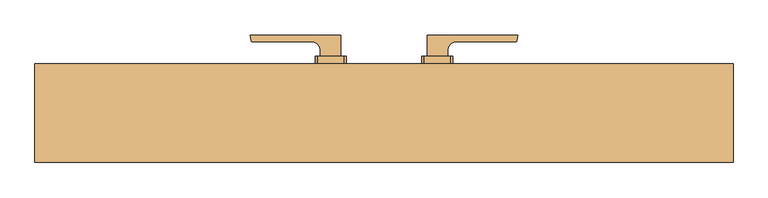
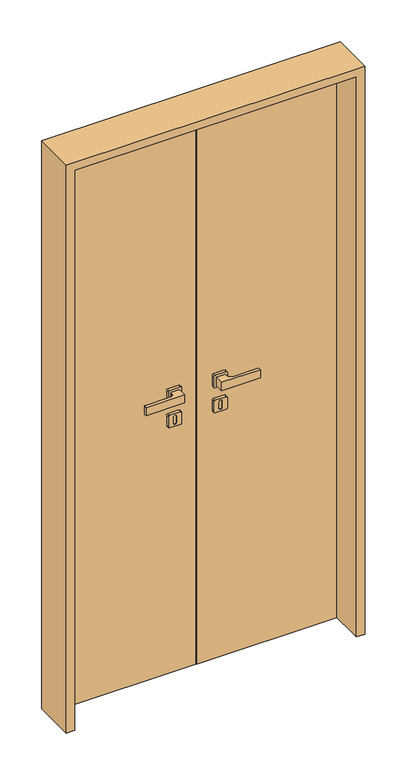
"""IFC4 building model written with IfcOpenShell, lengths in millimetres: door geometry, porta multiplas_growarq : porta giro duplo 50 cm_growarq."""

from ifc_helpers import new_model, si_unit, point, frame, frame_2d, origin, origin_with_axes, place, context, project, spatial, polyline, circle_curve, trimmed, segment, composite_curve, outline, extrude, source, transform, mapped, element, save
from ifc_brep_helpers import plane_surface, cylinder_surface, revolved_surface, advanced_brep


def door_77e2ac2a(model_context):
    return source(origin(), model_context, "Body", "SolidModel", [
        advanced_brep(
        [(-61.4752094, 86.0, 975.2140175), (-57.4752094, 86.0, 971.2140175), (-57.4752094, 86.0, 932.3348635), (-61.4752094, 86.0, 928.3348635), (-100.524804, 86.0, 928.3348635), (-104.524804, 86.0, 932.3348635), (-104.524804, 86.0, 971.2071442), (-100.5179308, 86.0, 975.2140175), (-75.9963765, 86.0, 963.1453546), (-86.0064486, 86.0, 963.1453546), (-86.0064486, 86.0, 940.4035264), (-75.9963765, 86.0, 940.4035264), (-61.4752094, 75.0, 975.2140175), (-100.5179308, 75.0, 975.2140175), (-104.524804, 75.0, 971.2071442), (-104.524804, 75.0, 932.3348635), (-100.524804, 75.0, 928.3348635), (-61.4752094, 75.0, 928.3348635), (-57.4752094, 75.0, 932.3348635), (-57.4752094, 75.0, 971.2140175), (-75.9963765, 84.0, 940.4035264), (-86.0064486, 84.0, 940.4035264), (-86.0064486, 84.0, 963.1453546), (-75.9963765, 84.0, 963.1453546)],
        [
            (0, 1, circle_curve(frame((-61.4752094, 86.0, 971.2140175), z_axis=(0.0, 1.0, 0.0), x_axis=(1.0, 0.0, 0.0)), 4.0)),
            (1, 2),
            (2, 3, circle_curve(frame((-61.4752094, 86.0, 932.3348635), z_axis=(0.0, 1.0, 0.0), x_axis=(1.0, 0.0, 0.0)), 4.0)),
            (3, 4),
            (4, 5, circle_curve(frame((-100.524804, 86.0, 932.3348635), z_axis=(0.0, 1.0, 0.0), x_axis=(1.0, 0.0, 0.0)), 4.0)),
            (5, 6),
            (6, 7, circle_curve(frame((-100.5179308, 86.0, 971.2071442), z_axis=(0.0, 1.0, 0.0), x_axis=(1.0, 0.0, 0.0)), 4.0068732)),
            (7, 0),
            (8, 9, circle_curve(frame((-81.0014126, 86.0, 963.1453546), z_axis=(0.0, -1.0, 0.0), x_axis=(1.0, 0.0, 0.0)), 5.0050361)),
            (9, 10),
            (10, 11, circle_curve(frame((-81.0014126, 86.0, 940.4035264), z_axis=(0.0, -1.0, 0.0), x_axis=(1.0, 0.0, 0.0)), 5.0050361)),
            (11, 8),
            (12, 13),
            (13, 14, circle_curve(frame((-100.5179308, 75.0, 971.2071442), z_axis=(0.0, -1.0, 0.0), x_axis=(1.0, 0.0, 0.0)), 4.0068732)),
            (14, 15),
            (15, 16, circle_curve(frame((-100.524804, 75.0, 932.3348635), z_axis=(0.0, -1.0, 0.0), x_axis=(1.0, 0.0, 0.0)), 4.0)),
            (16, 17),
            (17, 18, circle_curve(frame((-61.4752094, 75.0, 932.3348635), z_axis=(0.0, -1.0, 0.0), x_axis=(1.0, 0.0, 0.0)), 4.0)),
            (18, 19),
            (19, 12, circle_curve(frame((-61.4752094, 75.0, 971.2140175), z_axis=(0.0, -1.0, 0.0), x_axis=(1.0, 0.0, 0.0)), 4.0)),
            (7, 13),
            (12, 0),
            (6, 14),
            (5, 15),
            (4, 16),
            (3, 17),
            (2, 18),
            (1, 19),
            (20, 21, circle_curve(frame((-81.0014126, 84.0, 940.4035264), z_axis=(0.0, 1.0, 0.0), x_axis=(1.0, 0.0, 0.0)), 5.0050361)),
            (21, 22),
            (22, 23, circle_curve(frame((-81.0014126, 84.0, 963.1453546), z_axis=(0.0, 1.0, 0.0), x_axis=(1.0, 0.0, 0.0)), 5.0050361)),
            (23, 20),
            (23, 8),
            (11, 20),
            (21, 10),
            (9, 22),
        ],
        [
            plane_surface(frame((-100.5218961, 86.0, 975.2140175), z_axis=(0.0, 1.0, 0.0), x_axis=(-1.0, 0.0, 0.0))),
            plane_surface(frame((-100.5218961, 75.0, 975.2140175), z_axis=(0.0, -1.0, 0.0), x_axis=(1.0, 0.0, 0.0))),
            plane_surface(frame((-61.4752094, 86.0, 975.2140175), z_axis=(0.0, 0.0, 1.0), x_axis=(0.0, -1.0, 0.0))),
            cylinder_surface(frame((-100.5179308, 75.0, 971.2071442), z_axis=(0.0, 1.0, 0.0), x_axis=(1.0, 0.0, 0.0)), 4.0068732),
            plane_surface(frame((-104.524804, 86.0, 971.2071442), z_axis=(-1.0, 0.0, 0.0), x_axis=(0.0, -1.0, 0.0))),
            cylinder_surface(frame((-100.524804, 75.0, 932.3348635), z_axis=(0.0, 1.0, 0.0), x_axis=(1.0, 0.0, 0.0)), 4.0),
            plane_surface(frame((-100.524804, 86.0, 928.3348635), z_axis=(0.0, 0.0, -1.0), x_axis=(0.0, -1.0, 0.0))),
            cylinder_surface(frame((-61.4752094, 75.0, 932.3348635), z_axis=(0.0, 1.0, 0.0), x_axis=(1.0, 0.0, 0.0)), 4.0),
            plane_surface(frame((-57.4752094, 86.0, 932.3348635), z_axis=(1.0, 0.0, 0.0), x_axis=(0.0, -1.0, 0.0))),
            cylinder_surface(frame((-61.4752094, 75.0, 971.2140175), z_axis=(0.0, 1.0, 0.0), x_axis=(1.0, 0.0, 0.0)), 4.0),
            plane_surface(frame((-75.9963765, 84.0, 952.9958878), z_axis=(0.0, 1.0, 0.0), x_axis=(0.0, 0.0, -1.0))),
            plane_surface(frame((-75.9963765, 86.0, 940.4035264), z_axis=(-1.0, 0.0, 0.0), x_axis=(0.0, -1.0, 0.0))),
            plane_surface(frame((-86.0064486, 86.0, 963.1453546), z_axis=(1.0, 0.0, 0.0), x_axis=(0.0, -1.0, 0.0))),
            revolved_surface(polyline([(-75.9963765, 86.0, 940.4035264), (-75.9963765, 84.0, 940.4035264)]), (-81.0014126, 84.0, 940.4035264), (0.0, 1.0, 0.0)),
            revolved_surface(polyline([(-75.9963765, 86.0, 963.1453546), (-75.9963765, 84.0, 963.1453546)]), (-81.0014126, 84.0, 963.1453546), (0.0, 1.0, 0.0)),
        ],
        [
            (0, [[1, 2, 3, 4, 5, 6, 7, 8], [9, 10, 11, 12]]),
            (1, [[13, 14, 15, 16, 17, 18, 19, 20]]),
            (2, [[21, -13, 22, -8]]),
            (3, [[23, -14, -21, -7]]),
            (4, [[24, -15, -23, -6]]),
            (5, [[25, -16, -24, -5]]),
            (6, [[26, -17, -25, -4]]),
            (7, [[27, -18, -26, -3]]),
            (8, [[28, -19, -27, -2]]),
            (9, [[-22, -20, -28, -1]]),
            (10, [[29, 30, 31, 32]]),
            (11, [[33, -12, 34, -32]]),
            (12, [[35, -10, 36, -30]]),
            (13, [[-34, -11, -35, -29]]),
            (14, [[-36, -9, -33, -31]]),
        ],
    ),
        advanced_brep(
        [(-61.4752094, 86.0, 1068.227973), (-57.4752094, 86.0, 1064.227973), (-57.4752094, 86.0, 1025.3488191), (-61.4752094, 86.0, 1021.3488191), (-100.524804, 86.0, 1021.3488191), (-104.524804, 86.0, 1025.3488191), (-104.524804, 86.0, 1064.2210998), (-100.5179308, 86.0, 1068.227973), (-61.4752094, 75.0, 1068.227973), (-100.5179308, 75.0, 1068.227973), (-104.524804, 75.0, 1064.2210998), (-104.524804, 75.0, 1025.3488191), (-100.524804, 75.0, 1021.3488191), (-61.4752094, 75.0, 1021.3488191), (-57.4752094, 75.0, 1025.3488191), (-57.4752094, 75.0, 1064.227973)],
        [
            (0, 1, circle_curve(frame((-61.4752094, 86.0, 1064.227973), z_axis=(0.0, 1.0, 0.0), x_axis=(1.0, 0.0, 0.0)), 4.0)),
            (1, 2),
            (2, 3, circle_curve(frame((-61.4752094, 86.0, 1025.3488191), z_axis=(0.0, 1.0, 0.0), x_axis=(1.0, 0.0, 0.0)), 4.0)),
            (3, 4),
            (4, 5, circle_curve(frame((-100.524804, 86.0, 1025.3488191), z_axis=(0.0, 1.0, 0.0), x_axis=(1.0, 0.0, 0.0)), 4.0)),
            (5, 6),
            (6, 7, circle_curve(frame((-100.5179308, 86.0, 1064.2210998), z_axis=(0.0, 1.0, 0.0), x_axis=(1.0, 0.0, 0.0)), 4.0068732)),
            (7, 0),
            (8, 9),
            (9, 10, circle_curve(frame((-100.5179308, 75.0, 1064.2210998), z_axis=(0.0, -1.0, 0.0), x_axis=(1.0, 0.0, 0.0)), 4.0068732)),
            (10, 11),
            (11, 12, circle_curve(frame((-100.524804, 75.0, 1025.3488191), z_axis=(0.0, -1.0, 0.0), x_axis=(1.0, 0.0, 0.0)), 4.0)),
            (12, 13),
            (13, 14, circle_curve(frame((-61.4752094, 75.0, 1025.3488191), z_axis=(0.0, -1.0, 0.0), x_axis=(1.0, 0.0, 0.0)), 4.0)),
            (14, 15),
            (15, 8, circle_curve(frame((-61.4752094, 75.0, 1064.227973), z_axis=(0.0, -1.0, 0.0), x_axis=(1.0, 0.0, 0.0)), 4.0)),
            (7, 9),
            (8, 0),
            (6, 10),
            (5, 11),
            (4, 12),
            (3, 13),
            (2, 14),
            (1, 15),
        ],
        [
            plane_surface(frame((-100.5218961, 86.0, 975.2140175), z_axis=(0.0, 1.0, 0.0), x_axis=(-1.0, 0.0, 0.0))),
            plane_surface(frame((-100.5218961, 75.0, 975.2140175), z_axis=(0.0, -1.0, 0.0), x_axis=(1.0, 0.0, 0.0))),
            plane_surface(frame((-61.4752094, 86.0, 1068.227973), z_axis=(0.0, 0.0, 1.0), x_axis=(0.0, -1.0, 0.0))),
            cylinder_surface(frame((-100.5179308, 75.0, 1064.2210998), z_axis=(0.0, 1.0, 0.0), x_axis=(1.0, 0.0, 0.0)), 4.0068732),
            plane_surface(frame((-104.524804, 86.0, 1064.2210998), z_axis=(-1.0, 0.0, 0.0), x_axis=(0.0, -1.0, 0.0))),
            cylinder_surface(frame((-100.524804, 75.0, 1025.3488191), z_axis=(0.0, 1.0, 0.0), x_axis=(1.0, 0.0, 0.0)), 4.0),
            plane_surface(frame((-100.524804, 86.0, 1021.3488191), z_axis=(0.0, 0.0, -1.0), x_axis=(0.0, -1.0, 0.0))),
            cylinder_surface(frame((-61.4752094, 75.0, 1025.3488191), z_axis=(0.0, 1.0, 0.0), x_axis=(1.0, 0.0, 0.0)), 4.0),
            plane_surface(frame((-57.4752094, 86.0, 1025.3488191), z_axis=(1.0, 0.0, 0.0), x_axis=(0.0, -1.0, 0.0))),
            cylinder_surface(frame((-61.4752094, 75.0, 1064.227973), z_axis=(0.0, 1.0, 0.0), x_axis=(1.0, 0.0, 0.0)), 4.0),
        ],
        [
            (0, [[1, 2, 3, 4, 5, 6, 7, 8]]),
            (1, [[9, 10, 11, 12, 13, 14, 15, 16]]),
            (2, [[17, -9, 18, -8]]),
            (3, [[19, -10, -17, -7]]),
            (4, [[20, -11, -19, -6]]),
            (5, [[21, -12, -20, -5]]),
            (6, [[22, -13, -21, -4]]),
            (7, [[23, -14, -22, -3]]),
            (8, [[24, -15, -23, -2]]),
            (9, [[-18, -16, -24, -1]]),
        ],
    ),
        extrude(outline(composite_curve([segment(polyline([(-65.4752094, 118.5150355), (-65.4752094, 86.7793682), (-96.524804, 86.7793682), (-96.524804, 93.5981558)]), True, "CONTINUOUS"), segment(trimmed(circle_curve(frame_2d((-111.5516421, 93.5981558)), 15.0268381), [point((-96.524804, 93.5981558))], [point((-111.5516421, 108.6249939))], True, "CARTESIAN"), True, "CONTINUOUS"), segment(polyline([(-111.5516421, 108.6249939), (-200.8409795, 108.6249939)]), True, "CONTINUOUS"), segment(trimmed(circle_curve(frame_2d((-200.8409795, 109.6372538)), 1.0122598), [point((-200.8409795, 108.6249939))], [point((-201.8378608, 109.4614767))], False, "CARTESIAN"), True, "CONTINUOUS"), segment(polyline([(-201.8378608, 109.4614767), (-203.4342475, 118.5150355), (-65.4752094, 118.5150355)]), True, "CONTINUOUS")], self_intersect=False)), frame((0.0, 0.0, 1029.3488191), z_axis=(0.0, 0.0, 1.0), x_axis=(1.0, 0.0, 0.0)), (0.0, 0.0, 1.0), 30.8791539),
        advanced_brep(
        [(-61.4752094, 34.0, 975.2140175), (-100.5179308, 34.0, 975.2140175), (-104.524804, 34.0, 971.2071442), (-104.524804, 34.0, 932.3348635), (-100.524804, 34.0, 928.3348635), (-61.4752094, 34.0, 928.3348635), (-57.4752094, 34.0, 932.3348635), (-57.4752094, 34.0, 971.2140175), (-75.9963765, 34.0, 963.1453546), (-75.9963765, 34.0, 940.4035264), (-86.0064486, 34.0, 940.4035264), (-86.0064486, 34.0, 963.1453546), (-61.4752094, 45.0, 975.2140175), (-57.4752094, 45.0, 971.2140175), (-57.4752094, 45.0, 932.3348635), (-61.4752094, 45.0, 928.3348635), (-100.524804, 45.0, 928.3348635), (-104.524804, 45.0, 932.3348635), (-104.524804, 45.0, 971.2071442), (-100.5179308, 45.0, 975.2140175), (-75.9963765, 36.0, 940.4035264), (-75.9963765, 36.0, 963.1453546), (-86.0064486, 36.0, 963.1453546), (-86.0064486, 36.0, 940.4035264)],
        [
            (0, 1),
            (1, 2, circle_curve(frame((-100.5179308, 34.0, 971.2071442), z_axis=(0.0, -1.0, 0.0), x_axis=(1.0, 0.0, 0.0)), 4.0068732)),
            (2, 3),
            (3, 4, circle_curve(frame((-100.524804, 34.0, 932.3348635), z_axis=(0.0, -1.0, 0.0), x_axis=(1.0, 0.0, 0.0)), 4.0)),
            (4, 5),
            (5, 6, circle_curve(frame((-61.4752094, 34.0, 932.3348635), z_axis=(0.0, -1.0, 0.0), x_axis=(1.0, 0.0, 0.0)), 4.0)),
            (6, 7),
            (7, 0, circle_curve(frame((-61.4752094, 34.0, 971.2140175), z_axis=(0.0, -1.0, 0.0), x_axis=(1.0, 0.0, 0.0)), 4.0)),
            (8, 9),
            (9, 10, circle_curve(frame((-81.0014126, 34.0, 940.4035264), z_axis=(0.0, 1.0, 0.0), x_axis=(1.0, 0.0, 0.0)), 5.0050361)),
            (10, 11),
            (11, 8, circle_curve(frame((-81.0014126, 34.0, 963.1453546), z_axis=(0.0, 1.0, 0.0), x_axis=(1.0, 0.0, 0.0)), 5.0050361)),
            (12, 13, circle_curve(frame((-61.4752094, 45.0, 971.2140175), z_axis=(0.0, 1.0, 0.0), x_axis=(1.0, 0.0, 0.0)), 4.0)),
            (13, 14),
            (14, 15, circle_curve(frame((-61.4752094, 45.0, 932.3348635), z_axis=(0.0, 1.0, 0.0), x_axis=(1.0, 0.0, 0.0)), 4.0)),
            (15, 16),
            (16, 17, circle_curve(frame((-100.524804, 45.0, 932.3348635), z_axis=(0.0, 1.0, 0.0), x_axis=(1.0, 0.0, 0.0)), 4.0)),
            (17, 18),
            (18, 19, circle_curve(frame((-100.5179308, 45.0, 971.2071442), z_axis=(0.0, 1.0, 0.0), x_axis=(1.0, 0.0, 0.0)), 4.0068732)),
            (19, 12),
            (0, 12),
            (19, 1),
            (18, 2),
            (17, 3),
            (16, 4),
            (15, 5),
            (14, 6),
            (13, 7),
            (20, 21),
            (21, 22, circle_curve(frame((-81.0014126, 36.0, 963.1453546), z_axis=(0.0, -1.0, 0.0), x_axis=(1.0, 0.0, 0.0)), 5.0050361)),
            (22, 23),
            (23, 20, circle_curve(frame((-81.0014126, 36.0, 940.4035264), z_axis=(0.0, -1.0, 0.0), x_axis=(1.0, 0.0, 0.0)), 5.0050361)),
            (20, 9),
            (8, 21),
            (22, 11),
            (10, 23),
        ],
        [
            plane_surface(frame((-100.5218961, 34.0, 975.2140175), z_axis=(0.0, -1.0, 0.0), x_axis=(-1.0, 0.0, 0.0))),
            plane_surface(frame((-100.5218961, 45.0, 975.2140175), z_axis=(0.0, 1.0, 0.0), x_axis=(1.0, 0.0, 0.0))),
            plane_surface(frame((-61.4752094, 34.0, 975.2140175), z_axis=(0.0, 0.0, 1.0), x_axis=(0.0, 1.0, 0.0))),
            cylinder_surface(frame((-100.5179308, 45.0, 971.2071442), z_axis=(0.0, -1.0, 0.0), x_axis=(1.0, 0.0, 0.0)), 4.0068732),
            plane_surface(frame((-104.524804, 34.0, 971.2071442), z_axis=(-1.0, 0.0, 0.0), x_axis=(0.0, 1.0, 0.0))),
            cylinder_surface(frame((-100.524804, 45.0, 932.3348635), z_axis=(0.0, -1.0, 0.0), x_axis=(1.0, 0.0, 0.0)), 4.0),
            plane_surface(frame((-100.524804, 34.0, 928.3348635), z_axis=(0.0, 0.0, -1.0), x_axis=(0.0, 1.0, 0.0))),
            cylinder_surface(frame((-61.4752094, 45.0, 932.3348635), z_axis=(0.0, -1.0, 0.0), x_axis=(1.0, 0.0, 0.0)), 4.0),
            plane_surface(frame((-57.4752094, 34.0, 932.3348635), z_axis=(1.0, 0.0, 0.0), x_axis=(0.0, 1.0, 0.0))),
            cylinder_surface(frame((-61.4752094, 45.0, 971.2140175), z_axis=(0.0, -1.0, 0.0), x_axis=(1.0, 0.0, 0.0)), 4.0),
            plane_surface(frame((-75.9963765, 36.0, 952.9958878), z_axis=(0.0, -1.0, 0.0), x_axis=(0.0, 0.0, -1.0))),
            plane_surface(frame((-75.9963765, 34.0, 940.4035264), z_axis=(-1.0, 0.0, 0.0), x_axis=(0.0, 1.0, 0.0))),
            plane_surface(frame((-86.0064486, 34.0, 963.1453546), z_axis=(1.0, 0.0, 0.0), x_axis=(0.0, 1.0, 0.0))),
            revolved_surface(polyline([(-75.9963765, 34.0, 940.4035264), (-75.9963765, 36.0, 940.4035264)]), (-81.0014126, 36.0, 940.4035264), (0.0, -1.0, 0.0)),
            revolved_surface(polyline([(-75.9963765, 34.0, 963.1453546), (-75.9963765, 36.0, 963.1453546)]), (-81.0014126, 36.0, 963.1453546), (0.0, -1.0, 0.0)),
        ],
        [
            (0, [[1, 2, 3, 4, 5, 6, 7, 8], [9, 10, 11, 12]]),
            (1, [[13, 14, 15, 16, 17, 18, 19, 20]]),
            (2, [[-1, 21, -20, 22]]),
            (3, [[-2, -22, -19, 23]]),
            (4, [[-3, -23, -18, 24]]),
            (5, [[-4, -24, -17, 25]]),
            (6, [[-5, -25, -16, 26]]),
            (7, [[-6, -26, -15, 27]]),
            (8, [[-7, -27, -14, 28]]),
            (9, [[-8, -28, -13, -21]]),
            (10, [[29, 30, 31, 32]]),
            (11, [[-29, 33, -9, 34]]),
            (12, [[-31, 35, -11, 36]]),
            (13, [[-32, -36, -10, -33]]),
            (14, [[-30, -34, -12, -35]]),
        ],
    ),
        advanced_brep(
        [(-61.4752094, 34.0, 1068.227973), (-100.5179308, 34.0, 1068.227973), (-104.524804, 34.0, 1064.2210998), (-104.524804, 34.0, 1025.3488191), (-100.524804, 34.0, 1021.3488191), (-61.4752094, 34.0, 1021.3488191), (-57.4752094, 34.0, 1025.3488191), (-57.4752094, 34.0, 1064.227973), (-61.4752094, 45.0, 1068.227973), (-57.4752094, 45.0, 1064.227973), (-57.4752094, 45.0, 1025.3488191), (-61.4752094, 45.0, 1021.3488191), (-100.524804, 45.0, 1021.3488191), (-104.524804, 45.0, 1025.3488191), (-104.524804, 45.0, 1064.2210998), (-100.5179308, 45.0, 1068.227973)],
        [
            (0, 1),
            (1, 2, circle_curve(frame((-100.5179308, 34.0, 1064.2210998), z_axis=(0.0, -1.0, 0.0), x_axis=(1.0, 0.0, 0.0)), 4.0068732)),
            (2, 3),
            (3, 4, circle_curve(frame((-100.524804, 34.0, 1025.3488191), z_axis=(0.0, -1.0, 0.0), x_axis=(1.0, 0.0, 0.0)), 4.0)),
            (4, 5),
            (5, 6, circle_curve(frame((-61.4752094, 34.0, 1025.3488191), z_axis=(0.0, -1.0, 0.0), x_axis=(1.0, 0.0, 0.0)), 4.0)),
            (6, 7),
            (7, 0, circle_curve(frame((-61.4752094, 34.0, 1064.227973), z_axis=(0.0, -1.0, 0.0), x_axis=(1.0, 0.0, 0.0)), 4.0)),
            (8, 9, circle_curve(frame((-61.4752094, 45.0, 1064.227973), z_axis=(0.0, 1.0, 0.0), x_axis=(1.0, 0.0, 0.0)), 4.0)),
            (9, 10),
            (10, 11, circle_curve(frame((-61.4752094, 45.0, 1025.3488191), z_axis=(0.0, 1.0, 0.0), x_axis=(1.0, 0.0, 0.0)), 4.0)),
            (11, 12),
            (12, 13, circle_curve(frame((-100.524804, 45.0, 1025.3488191), z_axis=(0.0, 1.0, 0.0), x_axis=(1.0, 0.0, 0.0)), 4.0)),
            (13, 14),
            (14, 15, circle_curve(frame((-100.5179308, 45.0, 1064.2210998), z_axis=(0.0, 1.0, 0.0), x_axis=(1.0, 0.0, 0.0)), 4.0068732)),
            (15, 8),
            (0, 8),
            (15, 1),
            (14, 2),
            (13, 3),
            (12, 4),
            (11, 5),
            (10, 6),
            (9, 7),
        ],
        [
            plane_surface(frame((-100.5218961, 34.0, 975.2140175), z_axis=(0.0, -1.0, 0.0), x_axis=(-1.0, 0.0, 0.0))),
            plane_surface(frame((-100.5218961, 45.0, 975.2140175), z_axis=(0.0, 1.0, 0.0), x_axis=(1.0, 0.0, 0.0))),
            plane_surface(frame((-61.4752094, 34.0, 1068.227973), z_axis=(0.0, 0.0, 1.0), x_axis=(0.0, 1.0, 0.0))),
            cylinder_surface(frame((-100.5179308, 45.0, 1064.2210998), z_axis=(0.0, -1.0, 0.0), x_axis=(1.0, 0.0, 0.0)), 4.0068732),
            plane_surface(frame((-104.524804, 34.0, 1064.2210998), z_axis=(-1.0, 0.0, 0.0), x_axis=(0.0, 1.0, 0.0))),
            cylinder_surface(frame((-100.524804, 45.0, 1025.3488191), z_axis=(0.0, -1.0, 0.0), x_axis=(1.0, 0.0, 0.0)), 4.0),
            plane_surface(frame((-100.524804, 34.0, 1021.3488191), z_axis=(0.0, 0.0, -1.0), x_axis=(0.0, 1.0, 0.0))),
            cylinder_surface(frame((-61.4752094, 45.0, 1025.3488191), z_axis=(0.0, -1.0, 0.0), x_axis=(1.0, 0.0, 0.0)), 4.0),
            plane_surface(frame((-57.4752094, 34.0, 1025.3488191), z_axis=(1.0, 0.0, 0.0), x_axis=(0.0, 1.0, 0.0))),
            cylinder_surface(frame((-61.4752094, 45.0, 1064.227973), z_axis=(0.0, -1.0, 0.0), x_axis=(1.0, 0.0, 0.0)), 4.0),
        ],
        [
            (0, [[1, 2, 3, 4, 5, 6, 7, 8]]),
            (1, [[9, 10, 11, 12, 13, 14, 15, 16]]),
            (2, [[-1, 17, -16, 18]]),
            (3, [[-2, -18, -15, 19]]),
            (4, [[-3, -19, -14, 20]]),
            (5, [[-4, -20, -13, 21]]),
            (6, [[-5, -21, -12, 22]]),
            (7, [[-6, -22, -11, 23]]),
            (8, [[-7, -23, -10, 24]]),
            (9, [[-8, -24, -9, -17]]),
        ],
    ),
        extrude(outline(composite_curve([segment(polyline([(-65.4752094, 1.4849645), (-203.4342475, 1.4849645), (-201.8378608, 10.5385233)]), True, "CONTINUOUS"), segment(trimmed(circle_curve(frame_2d((-200.8409795, 10.3627462)), 1.0122598), [point((-201.8378608, 10.5385233))], [point((-200.8409795, 11.3750061))], False, "CARTESIAN"), True, "CONTINUOUS"), segment(polyline([(-200.8409795, 11.3750061), (-111.5516421, 11.3750061)]), True, "CONTINUOUS"), segment(trimmed(circle_curve(frame_2d((-111.5516421, 26.4018442)), 15.0268381), [point((-111.5516421, 11.3750061))], [point((-96.524804, 26.4018442))], True, "CARTESIAN"), True, "CONTINUOUS"), segment(polyline([(-96.524804, 26.4018442), (-96.524804, 33.2206318), (-65.4752094, 33.2206318), (-65.4752094, 1.4849645)]), True, "CONTINUOUS")], self_intersect=False)), frame((0.0, 0.0, 1029.3488191), z_axis=(0.0, 0.0, 1.0), x_axis=(1.0, 0.0, 0.0)), (0.0, 0.0, 1.0), 30.8791539),
        extrude(outline(polyline([(-1.0, 45.0), (-498.0, 45.0), (-498.0, 75.0), (-1.0, 75.0), (-1.0, 45.0)])), origin_with_axes(), (0.0, 0.0, 1.0), 2098.0),
        advanced_brep(
        [(61.4752094, 86.0, 975.2140175), (100.5179308, 86.0, 975.2140175), (104.524804, 86.0, 971.2071442), (104.524804, 86.0, 932.3348635), (100.524804, 86.0, 928.3348635), (61.4752094, 86.0, 928.3348635), (57.4752094, 86.0, 932.3348635), (57.4752094, 86.0, 971.2140175), (75.9963765, 86.0, 963.1453546), (75.9963765, 86.0, 940.4035264), (86.0064486, 86.0, 940.4035264), (86.0064486, 86.0, 963.1453546), (61.4752094, 75.0, 975.2140175), (57.4752094, 75.0, 971.2140175), (57.4752094, 75.0, 932.3348635), (61.4752094, 75.0, 928.3348635), (100.524804, 75.0, 928.3348635), (104.524804, 75.0, 932.3348635), (104.524804, 75.0, 971.2071442), (100.5179308, 75.0, 975.2140175), (75.9963765, 84.0, 940.4035264), (75.9963765, 84.0, 963.1453546), (86.0064486, 84.0, 963.1453546), (86.0064486, 84.0, 940.4035264)],
        [
            (0, 1),
            (1, 2, circle_curve(frame((100.5179308, 86.0, 971.2071442), z_axis=(0.0, 1.0, 0.0), x_axis=(-1.0, 0.0, 0.0)), 4.0068732)),
            (2, 3),
            (3, 4, circle_curve(frame((100.524804, 86.0, 932.3348635), z_axis=(0.0, 1.0, 0.0), x_axis=(-1.0, 0.0, 0.0)), 4.0)),
            (4, 5),
            (5, 6, circle_curve(frame((61.4752094, 86.0, 932.3348635), z_axis=(0.0, 1.0, 0.0), x_axis=(-1.0, 0.0, 0.0)), 4.0)),
            (6, 7),
            (7, 0, circle_curve(frame((61.4752094, 86.0, 971.2140175), z_axis=(0.0, 1.0, 0.0), x_axis=(-1.0, 0.0, 0.0)), 4.0)),
            (8, 9),
            (9, 10, circle_curve(frame((81.0014126, 86.0, 940.4035264), z_axis=(0.0, -1.0, 0.0), x_axis=(-1.0, 0.0, 0.0)), 5.0050361)),
            (10, 11),
            (11, 8, circle_curve(frame((81.0014126, 86.0, 963.1453546), z_axis=(0.0, -1.0, 0.0), x_axis=(-1.0, 0.0, 0.0)), 5.0050361)),
            (12, 13, circle_curve(frame((61.4752094, 75.0, 971.2140175), z_axis=(0.0, -1.0, 0.0), x_axis=(-1.0, 0.0, 0.0)), 4.0)),
            (13, 14),
            (14, 15, circle_curve(frame((61.4752094, 75.0, 932.3348635), z_axis=(0.0, -1.0, 0.0), x_axis=(-1.0, 0.0, 0.0)), 4.0)),
            (15, 16),
            (16, 17, circle_curve(frame((100.524804, 75.0, 932.3348635), z_axis=(0.0, -1.0, 0.0), x_axis=(-1.0, 0.0, 0.0)), 4.0)),
            (17, 18),
            (18, 19, circle_curve(frame((100.5179308, 75.0, 971.2071442), z_axis=(0.0, -1.0, 0.0), x_axis=(-1.0, 0.0, 0.0)), 4.0068732)),
            (19, 12),
            (0, 12),
            (19, 1),
            (18, 2),
            (17, 3),
            (16, 4),
            (15, 5),
            (14, 6),
            (13, 7),
            (20, 21),
            (21, 22, circle_curve(frame((81.0014126, 84.0, 963.1453546), z_axis=(0.0, 1.0, 0.0), x_axis=(-1.0, 0.0, 0.0)), 5.0050361)),
            (22, 23),
            (23, 20, circle_curve(frame((81.0014126, 84.0, 940.4035264), z_axis=(0.0, 1.0, 0.0), x_axis=(-1.0, 0.0, 0.0)), 5.0050361)),
            (20, 9),
            (8, 21),
            (22, 11),
            (10, 23),
        ],
        [
            plane_surface(frame((100.5218961, 86.0, 975.2140175), z_axis=(0.0, 1.0, 0.0), x_axis=(1.0, 0.0, 0.0))),
            plane_surface(frame((100.5218961, 75.0, 975.2140175), z_axis=(0.0, -1.0, 0.0), x_axis=(-1.0, 0.0, 0.0))),
            plane_surface(frame((61.4752094, 86.0, 975.2140175), z_axis=(0.0, 0.0, 1.0), x_axis=(0.0, -1.0, 0.0))),
            cylinder_surface(frame((100.5179308, 75.0, 971.2071442), z_axis=(0.0, 1.0, 0.0), x_axis=(-1.0, 0.0, 0.0)), 4.0068732),
            plane_surface(frame((104.524804, 86.0, 971.2071442), z_axis=(1.0, 0.0, 0.0), x_axis=(0.0, -1.0, 0.0))),
            cylinder_surface(frame((100.524804, 75.0, 932.3348635), z_axis=(0.0, 1.0, 0.0), x_axis=(-1.0, 0.0, 0.0)), 4.0),
            plane_surface(frame((100.524804, 86.0, 928.3348635), z_axis=(0.0, 0.0, -1.0), x_axis=(0.0, -1.0, 0.0))),
            cylinder_surface(frame((61.4752094, 75.0, 932.3348635), z_axis=(0.0, 1.0, 0.0), x_axis=(-1.0, 0.0, 0.0)), 4.0),
            plane_surface(frame((57.4752094, 86.0, 932.3348635), z_axis=(-1.0, 0.0, 0.0), x_axis=(0.0, -1.0, 0.0))),
            cylinder_surface(frame((61.4752094, 75.0, 971.2140175), z_axis=(0.0, 1.0, 0.0), x_axis=(-1.0, 0.0, 0.0)), 4.0),
            plane_surface(frame((75.9963765, 84.0, 952.9958878), z_axis=(0.0, 1.0, 0.0), x_axis=(0.0, 0.0, -1.0))),
            plane_surface(frame((75.9963765, 86.0, 940.4035264), z_axis=(1.0, 0.0, 0.0), x_axis=(0.0, -1.0, 0.0))),
            plane_surface(frame((86.0064486, 86.0, 963.1453546), z_axis=(-1.0, 0.0, 0.0), x_axis=(0.0, -1.0, 0.0))),
            revolved_surface(polyline([(75.9963765, 86.0, 940.4035264), (75.9963765, 84.0, 940.4035264)]), (81.0014126, 84.0, 940.4035264), (0.0, 1.0, 0.0)),
            revolved_surface(polyline([(75.9963765, 86.0, 963.1453546), (75.9963765, 84.0, 963.1453546)]), (81.0014126, 84.0, 963.1453546), (0.0, 1.0, 0.0)),
        ],
        [
            (0, [[1, 2, 3, 4, 5, 6, 7, 8], [9, 10, 11, 12]]),
            (1, [[13, 14, 15, 16, 17, 18, 19, 20]]),
            (2, [[-1, 21, -20, 22]]),
            (3, [[-2, -22, -19, 23]]),
            (4, [[-3, -23, -18, 24]]),
            (5, [[-4, -24, -17, 25]]),
            (6, [[-5, -25, -16, 26]]),
            (7, [[-6, -26, -15, 27]]),
            (8, [[-7, -27, -14, 28]]),
            (9, [[-8, -28, -13, -21]]),
            (10, [[29, 30, 31, 32]]),
            (11, [[-29, 33, -9, 34]]),
            (12, [[-31, 35, -11, 36]]),
            (13, [[-32, -36, -10, -33]]),
            (14, [[-30, -34, -12, -35]]),
        ],
    ),
        advanced_brep(
        [(61.4752094, 86.0, 1068.227973), (100.5179308, 86.0, 1068.227973), (104.524804, 86.0, 1064.2210998), (104.524804, 86.0, 1025.3488191), (100.524804, 86.0, 1021.3488191), (61.4752094, 86.0, 1021.3488191), (57.4752094, 86.0, 1025.3488191), (57.4752094, 86.0, 1064.227973), (61.4752094, 75.0, 1068.227973), (57.4752094, 75.0, 1064.227973), (57.4752094, 75.0, 1025.3488191), (61.4752094, 75.0, 1021.3488191), (100.524804, 75.0, 1021.3488191), (104.524804, 75.0, 1025.3488191), (104.524804, 75.0, 1064.2210998), (100.5179308, 75.0, 1068.227973)],
        [
            (0, 1),
            (1, 2, circle_curve(frame((100.5179308, 86.0, 1064.2210998), z_axis=(0.0, 1.0, 0.0), x_axis=(-1.0, 0.0, 0.0)), 4.0068732)),
            (2, 3),
            (3, 4, circle_curve(frame((100.524804, 86.0, 1025.3488191), z_axis=(0.0, 1.0, 0.0), x_axis=(-1.0, 0.0, 0.0)), 4.0)),
            (4, 5),
            (5, 6, circle_curve(frame((61.4752094, 86.0, 1025.3488191), z_axis=(0.0, 1.0, 0.0), x_axis=(-1.0, 0.0, 0.0)), 4.0)),
            (6, 7),
            (7, 0, circle_curve(frame((61.4752094, 86.0, 1064.227973), z_axis=(0.0, 1.0, 0.0), x_axis=(-1.0, 0.0, 0.0)), 4.0)),
            (8, 9, circle_curve(frame((61.4752094, 75.0, 1064.227973), z_axis=(0.0, -1.0, 0.0), x_axis=(-1.0, 0.0, 0.0)), 4.0)),
            (9, 10),
            (10, 11, circle_curve(frame((61.4752094, 75.0, 1025.3488191), z_axis=(0.0, -1.0, 0.0), x_axis=(-1.0, 0.0, 0.0)), 4.0)),
            (11, 12),
            (12, 13, circle_curve(frame((100.524804, 75.0, 1025.3488191), z_axis=(0.0, -1.0, 0.0), x_axis=(-1.0, 0.0, 0.0)), 4.0)),
            (13, 14),
            (14, 15, circle_curve(frame((100.5179308, 75.0, 1064.2210998), z_axis=(0.0, -1.0, 0.0), x_axis=(-1.0, 0.0, 0.0)), 4.0068732)),
            (15, 8),
            (0, 8),
            (15, 1),
            (14, 2),
            (13, 3),
            (12, 4),
            (11, 5),
            (10, 6),
            (9, 7),
        ],
        [
            plane_surface(frame((100.5218961, 86.0, 975.2140175), z_axis=(0.0, 1.0, 0.0), x_axis=(1.0, 0.0, 0.0))),
            plane_surface(frame((100.5218961, 75.0, 975.2140175), z_axis=(0.0, -1.0, 0.0), x_axis=(-1.0, 0.0, 0.0))),
            plane_surface(frame((61.4752094, 86.0, 1068.227973), z_axis=(0.0, 0.0, 1.0), x_axis=(0.0, -1.0, 0.0))),
            cylinder_surface(frame((100.5179308, 75.0, 1064.2210998), z_axis=(0.0, 1.0, 0.0), x_axis=(-1.0, 0.0, 0.0)), 4.0068732),
            plane_surface(frame((104.524804, 86.0, 1064.2210998), z_axis=(1.0, 0.0, 0.0), x_axis=(0.0, -1.0, 0.0))),
            cylinder_surface(frame((100.524804, 75.0, 1025.3488191), z_axis=(0.0, 1.0, 0.0), x_axis=(-1.0, 0.0, 0.0)), 4.0),
            plane_surface(frame((100.524804, 86.0, 1021.3488191), z_axis=(0.0, 0.0, -1.0), x_axis=(0.0, -1.0, 0.0))),
            cylinder_surface(frame((61.4752094, 75.0, 1025.3488191), z_axis=(0.0, 1.0, 0.0), x_axis=(-1.0, 0.0, 0.0)), 4.0),
            plane_surface(frame((57.4752094, 86.0, 1025.3488191), z_axis=(-1.0, 0.0, 0.0), x_axis=(0.0, -1.0, 0.0))),
            cylinder_surface(frame((61.4752094, 75.0, 1064.227973), z_axis=(0.0, 1.0, 0.0), x_axis=(-1.0, 0.0, 0.0)), 4.0),
        ],
        [
            (0, [[1, 2, 3, 4, 5, 6, 7, 8]]),
            (1, [[9, 10, 11, 12, 13, 14, 15, 16]]),
            (2, [[-1, 17, -16, 18]]),
            (3, [[-2, -18, -15, 19]]),
            (4, [[-3, -19, -14, 20]]),
            (5, [[-4, -20, -13, 21]]),
            (6, [[-5, -21, -12, 22]]),
            (7, [[-6, -22, -11, 23]]),
            (8, [[-7, -23, -10, 24]]),
            (9, [[-8, -24, -9, -17]]),
        ],
    ),
        extrude(outline(composite_curve([segment(polyline([(65.4752094, 118.5150355), (203.4342475, 118.5150355), (201.8378608, 109.4614767)]), True, "CONTINUOUS"), segment(trimmed(circle_curve(frame_2d((200.8409795, 109.6372538)), 1.0122598), [point((201.8378608, 109.4614767))], [point((200.8409795, 108.6249939))], False, "CARTESIAN"), True, "CONTINUOUS"), segment(polyline([(200.8409795, 108.6249939), (111.5516421, 108.6249939)]), True, "CONTINUOUS"), segment(trimmed(circle_curve(frame_2d((111.5516421, 93.5981558)), 15.0268381), [point((111.5516421, 108.6249939))], [point((96.524804, 93.5981558))], True, "CARTESIAN"), True, "CONTINUOUS"), segment(polyline([(96.524804, 93.5981558), (96.524804, 86.7793682), (65.4752094, 86.7793682), (65.4752094, 118.5150355)]), True, "CONTINUOUS")], self_intersect=False)), frame((0.0, 0.0, 1029.3488191), z_axis=(0.0, 0.0, 1.0), x_axis=(1.0, 0.0, 0.0)), (0.0, 0.0, 1.0), 30.8791539),
        advanced_brep(
        [(61.4752094, 34.0, 975.2140175), (57.4752094, 34.0, 971.2140175), (57.4752094, 34.0, 932.3348635), (61.4752094, 34.0, 928.3348635), (100.524804, 34.0, 928.3348635), (104.524804, 34.0, 932.3348635), (104.524804, 34.0, 971.2071442), (100.5179308, 34.0, 975.2140175), (75.9963765, 34.0, 963.1453546), (86.0064486, 34.0, 963.1453546), (86.0064486, 34.0, 940.4035264), (75.9963765, 34.0, 940.4035264), (61.4752094, 45.0, 975.2140175), (100.5179308, 45.0, 975.2140175), (104.524804, 45.0, 971.2071442), (104.524804, 45.0, 932.3348635), (100.524804, 45.0, 928.3348635), (61.4752094, 45.0, 928.3348635), (57.4752094, 45.0, 932.3348635), (57.4752094, 45.0, 971.2140175), (75.9963765, 36.0, 940.4035264), (86.0064486, 36.0, 940.4035264), (86.0064486, 36.0, 963.1453546), (75.9963765, 36.0, 963.1453546)],
        [
            (0, 1, circle_curve(frame((61.4752094, 34.0, 971.2140175), z_axis=(0.0, -1.0, 0.0), x_axis=(-1.0, 0.0, 0.0)), 4.0)),
            (1, 2),
            (2, 3, circle_curve(frame((61.4752094, 34.0, 932.3348635), z_axis=(0.0, -1.0, 0.0), x_axis=(-1.0, 0.0, 0.0)), 4.0)),
            (3, 4),
            (4, 5, circle_curve(frame((100.524804, 34.0, 932.3348635), z_axis=(0.0, -1.0, 0.0), x_axis=(-1.0, 0.0, 0.0)), 4.0)),
            (5, 6),
            (6, 7, circle_curve(frame((100.5179308, 34.0, 971.2071442), z_axis=(0.0, -1.0, 0.0), x_axis=(-1.0, 0.0, 0.0)), 4.0068732)),
            (7, 0),
            (8, 9, circle_curve(frame((81.0014126, 34.0, 963.1453546), z_axis=(0.0, 1.0, 0.0), x_axis=(-1.0, 0.0, 0.0)), 5.0050361)),
            (9, 10),
            (10, 11, circle_curve(frame((81.0014126, 34.0, 940.4035264), z_axis=(0.0, 1.0, 0.0), x_axis=(-1.0, 0.0, 0.0)), 5.0050361)),
            (11, 8),
            (12, 13),
            (13, 14, circle_curve(frame((100.5179308, 45.0, 971.2071442), z_axis=(0.0, 1.0, 0.0), x_axis=(-1.0, 0.0, 0.0)), 4.0068732)),
            (14, 15),
            (15, 16, circle_curve(frame((100.524804, 45.0, 932.3348635), z_axis=(0.0, 1.0, 0.0), x_axis=(-1.0, 0.0, 0.0)), 4.0)),
            (16, 17),
            (17, 18, circle_curve(frame((61.4752094, 45.0, 932.3348635), z_axis=(0.0, 1.0, 0.0), x_axis=(-1.0, 0.0, 0.0)), 4.0)),
            (18, 19),
            (19, 12, circle_curve(frame((61.4752094, 45.0, 971.2140175), z_axis=(0.0, 1.0, 0.0), x_axis=(-1.0, 0.0, 0.0)), 4.0)),
            (7, 13),
            (12, 0),
            (6, 14),
            (5, 15),
            (4, 16),
            (3, 17),
            (2, 18),
            (1, 19),
            (20, 21, circle_curve(frame((81.0014126, 36.0, 940.4035264), z_axis=(0.0, -1.0, 0.0), x_axis=(-1.0, 0.0, 0.0)), 5.0050361)),
            (21, 22),
            (22, 23, circle_curve(frame((81.0014126, 36.0, 963.1453546), z_axis=(0.0, -1.0, 0.0), x_axis=(-1.0, 0.0, 0.0)), 5.0050361)),
            (23, 20),
            (23, 8),
            (11, 20),
            (21, 10),
            (9, 22),
        ],
        [
            plane_surface(frame((100.5218961, 34.0, 975.2140175), z_axis=(0.0, -1.0, 0.0), x_axis=(1.0, 0.0, 0.0))),
            plane_surface(frame((100.5218961, 45.0, 975.2140175), z_axis=(0.0, 1.0, 0.0), x_axis=(-1.0, 0.0, 0.0))),
            plane_surface(frame((61.4752094, 34.0, 975.2140175), z_axis=(0.0, 0.0, 1.0), x_axis=(0.0, 1.0, 0.0))),
            cylinder_surface(frame((100.5179308, 45.0, 971.2071442), z_axis=(0.0, -1.0, 0.0), x_axis=(-1.0, 0.0, 0.0)), 4.0068732),
            plane_surface(frame((104.524804, 34.0, 971.2071442), z_axis=(1.0, 0.0, 0.0), x_axis=(0.0, 1.0, 0.0))),
            cylinder_surface(frame((100.524804, 45.0, 932.3348635), z_axis=(0.0, -1.0, 0.0), x_axis=(-1.0, 0.0, 0.0)), 4.0),
            plane_surface(frame((100.524804, 34.0, 928.3348635), z_axis=(0.0, 0.0, -1.0), x_axis=(0.0, 1.0, 0.0))),
            cylinder_surface(frame((61.4752094, 45.0, 932.3348635), z_axis=(0.0, -1.0, 0.0), x_axis=(-1.0, 0.0, 0.0)), 4.0),
            plane_surface(frame((57.4752094, 34.0, 932.3348635), z_axis=(-1.0, 0.0, 0.0), x_axis=(0.0, 1.0, 0.0))),
            cylinder_surface(frame((61.4752094, 45.0, 971.2140175), z_axis=(0.0, -1.0, 0.0), x_axis=(-1.0, 0.0, 0.0)), 4.0),
            plane_surface(frame((75.9963765, 36.0, 952.9958878), z_axis=(0.0, -1.0, 0.0), x_axis=(0.0, 0.0, -1.0))),
            plane_surface(frame((75.9963765, 34.0, 940.4035264), z_axis=(1.0, 0.0, 0.0), x_axis=(0.0, 1.0, 0.0))),
            plane_surface(frame((86.0064486, 34.0, 963.1453546), z_axis=(-1.0, 0.0, 0.0), x_axis=(0.0, 1.0, 0.0))),
            revolved_surface(polyline([(75.9963765, 34.0, 940.4035264), (75.9963765, 36.0, 940.4035264)]), (81.0014126, 36.0, 940.4035264), (0.0, -1.0, 0.0)),
            revolved_surface(polyline([(75.9963765, 34.0, 963.1453546), (75.9963765, 36.0, 963.1453546)]), (81.0014126, 36.0, 963.1453546), (0.0, -1.0, 0.0)),
        ],
        [
            (0, [[1, 2, 3, 4, 5, 6, 7, 8], [9, 10, 11, 12]]),
            (1, [[13, 14, 15, 16, 17, 18, 19, 20]]),
            (2, [[21, -13, 22, -8]]),
            (3, [[23, -14, -21, -7]]),
            (4, [[24, -15, -23, -6]]),
            (5, [[25, -16, -24, -5]]),
            (6, [[26, -17, -25, -4]]),
            (7, [[27, -18, -26, -3]]),
            (8, [[28, -19, -27, -2]]),
            (9, [[-22, -20, -28, -1]]),
            (10, [[29, 30, 31, 32]]),
            (11, [[33, -12, 34, -32]]),
            (12, [[35, -10, 36, -30]]),
            (13, [[-34, -11, -35, -29]]),
            (14, [[-36, -9, -33, -31]]),
        ],
    ),
        advanced_brep(
        [(61.4752094, 34.0, 1068.227973), (57.4752094, 34.0, 1064.227973), (57.4752094, 34.0, 1025.3488191), (61.4752094, 34.0, 1021.3488191), (100.524804, 34.0, 1021.3488191), (104.524804, 34.0, 1025.3488191), (104.524804, 34.0, 1064.2210998), (100.5179308, 34.0, 1068.227973), (61.4752094, 45.0, 1068.227973), (100.5179308, 45.0, 1068.227973), (104.524804, 45.0, 1064.2210998), (104.524804, 45.0, 1025.3488191), (100.524804, 45.0, 1021.3488191), (61.4752094, 45.0, 1021.3488191), (57.4752094, 45.0, 1025.3488191), (57.4752094, 45.0, 1064.227973)],
        [
            (0, 1, circle_curve(frame((61.4752094, 34.0, 1064.227973), z_axis=(0.0, -1.0, 0.0), x_axis=(-1.0, 0.0, 0.0)), 4.0)),
            (1, 2),
            (2, 3, circle_curve(frame((61.4752094, 34.0, 1025.3488191), z_axis=(0.0, -1.0, 0.0), x_axis=(-1.0, 0.0, 0.0)), 4.0)),
            (3, 4),
            (4, 5, circle_curve(frame((100.524804, 34.0, 1025.3488191), z_axis=(0.0, -1.0, 0.0), x_axis=(-1.0, 0.0, 0.0)), 4.0)),
            (5, 6),
            (6, 7, circle_curve(frame((100.5179308, 34.0, 1064.2210998), z_axis=(0.0, -1.0, 0.0), x_axis=(-1.0, 0.0, 0.0)), 4.0068732)),
            (7, 0),
            (8, 9),
            (9, 10, circle_curve(frame((100.5179308, 45.0, 1064.2210998), z_axis=(0.0, 1.0, 0.0), x_axis=(-1.0, 0.0, 0.0)), 4.0068732)),
            (10, 11),
            (11, 12, circle_curve(frame((100.524804, 45.0, 1025.3488191), z_axis=(0.0, 1.0, 0.0), x_axis=(-1.0, 0.0, 0.0)), 4.0)),
            (12, 13),
            (13, 14, circle_curve(frame((61.4752094, 45.0, 1025.3488191), z_axis=(0.0, 1.0, 0.0), x_axis=(-1.0, 0.0, 0.0)), 4.0)),
            (14, 15),
            (15, 8, circle_curve(frame((61.4752094, 45.0, 1064.227973), z_axis=(0.0, 1.0, 0.0), x_axis=(-1.0, 0.0, 0.0)), 4.0)),
            (7, 9),
            (8, 0),
            (6, 10),
            (5, 11),
            (4, 12),
            (3, 13),
            (2, 14),
            (1, 15),
        ],
        [
            plane_surface(frame((100.5218961, 34.0, 975.2140175), z_axis=(0.0, -1.0, 0.0), x_axis=(1.0, 0.0, 0.0))),
            plane_surface(frame((100.5218961, 45.0, 975.2140175), z_axis=(0.0, 1.0, 0.0), x_axis=(-1.0, 0.0, 0.0))),
            plane_surface(frame((61.4752094, 34.0, 1068.227973), z_axis=(0.0, 0.0, 1.0), x_axis=(0.0, 1.0, 0.0))),
            cylinder_surface(frame((100.5179308, 45.0, 1064.2210998), z_axis=(0.0, -1.0, 0.0), x_axis=(-1.0, 0.0, 0.0)), 4.0068732),
            plane_surface(frame((104.524804, 34.0, 1064.2210998), z_axis=(1.0, 0.0, 0.0), x_axis=(0.0, 1.0, 0.0))),
            cylinder_surface(frame((100.524804, 45.0, 1025.3488191), z_axis=(0.0, -1.0, 0.0), x_axis=(-1.0, 0.0, 0.0)), 4.0),
            plane_surface(frame((100.524804, 34.0, 1021.3488191), z_axis=(0.0, 0.0, -1.0), x_axis=(0.0, 1.0, 0.0))),
            cylinder_surface(frame((61.4752094, 45.0, 1025.3488191), z_axis=(0.0, -1.0, 0.0), x_axis=(-1.0, 0.0, 0.0)), 4.0),
            plane_surface(frame((57.4752094, 34.0, 1025.3488191), z_axis=(-1.0, 0.0, 0.0), x_axis=(0.0, 1.0, 0.0))),
            cylinder_surface(frame((61.4752094, 45.0, 1064.227973), z_axis=(0.0, -1.0, 0.0), x_axis=(-1.0, 0.0, 0.0)), 4.0),
        ],
        [
            (0, [[1, 2, 3, 4, 5, 6, 7, 8]]),
            (1, [[9, 10, 11, 12, 13, 14, 15, 16]]),
            (2, [[17, -9, 18, -8]]),
            (3, [[19, -10, -17, -7]]),
            (4, [[20, -11, -19, -6]]),
            (5, [[21, -12, -20, -5]]),
            (6, [[22, -13, -21, -4]]),
            (7, [[23, -14, -22, -3]]),
            (8, [[24, -15, -23, -2]]),
            (9, [[-18, -16, -24, -1]]),
        ],
    ),
        extrude(outline(composite_curve([segment(polyline([(65.4752094, 1.4849645), (65.4752094, 33.2206318), (96.524804, 33.2206318), (96.524804, 26.4018442)]), True, "CONTINUOUS"), segment(trimmed(circle_curve(frame_2d((111.5516421, 26.4018442)), 15.0268381), [point((96.524804, 26.4018442))], [point((111.5516421, 11.3750061))], True, "CARTESIAN"), True, "CONTINUOUS"), segment(polyline([(111.5516421, 11.3750061), (200.8409795, 11.3750061)]), True, "CONTINUOUS"), segment(trimmed(circle_curve(frame_2d((200.8409795, 10.3627462)), 1.0122598), [point((200.8409795, 11.3750061))], [point((201.8378608, 10.5385233))], False, "CARTESIAN"), True, "CONTINUOUS"), segment(polyline([(201.8378608, 10.5385233), (203.4342475, 1.4849645), (65.4752094, 1.4849645)]), True, "CONTINUOUS")], self_intersect=False)), frame((0.0, 0.0, 1029.3488191), z_axis=(0.0, 0.0, 1.0), x_axis=(1.0, 0.0, 0.0)), (0.0, 0.0, 1.0), 30.8791539),
        extrude(outline(polyline([(1.0, 45.0), (1.0, 75.0), (498.0, 75.0), (498.0, 45.0), (1.0, 45.0)])), origin_with_axes(), (0.0, 0.0, 1.0), 2098.0),
        extrude(outline(polyline([(0.0, 500.0), (0.0, 530.0), (2130.0, 530.0), (2130.0, -530.0), (0.0, -530.0), (0.0, -500.0), (2100.0, -500.0), (2100.0, 500.0), (0.0, 500.0)])), frame((0.0, -75.0, 0.0), z_axis=(0.0, 1.0, 0.0), x_axis=(0.0, 0.0, 1.0)), (0.0, 0.0, 1.0), 150.0),
    ])


if __name__ == "__main__":
    model = new_model("IFC4")
    model_context = context("Model", 3, world=origin())
    ifc_project = project(units=[si_unit("LENGTHUNIT", "METRE", prefix="MILLI")], contexts=[model_context])
    site = spatial("IfcSite", under=ifc_project)
    building = spatial("IfcBuilding", under=site)
    placement = place(None, origin())
    door_shape = door_77e2ac2a(model_context)
    element("IfcDoor", 1, ObjectType="porta multiplas_growarq : porta giro duplo 50 cm_growarq", at=placement, inside=building, context=model_context, shape_type="MappedRepresentation", body=[
        mapped(door_shape, transform((0.0, 0.0, 0.0), x_axis=(1.0, 0.0, 0.0), y_axis=(0.0, 1.0, 0.0), z_axis=(0.0, 0.0, 1.0))),
    ])
    save(model, "model.ifc")

# Revit data of these elements
# Type "porta multiplas_growarq : porta giro duplo 50 cm_growarq"
#   Type Mark = "C28"
#   Description = "Porta de Madeira com uma folha de abrir"
#   Analytic Construction = "<None>"
#   Rough Width = 1060 mm
#   Largura Guarnição = 75 mm
#   Espessura Guarnição = 10 mm
#   Thickness = 30 mm
#   Rough Height = 2130 mm
#   Marco = 30 mm
#   Largura Folha Eixo = 796 mm
#   Height = 2100 mm
#   Width = 1000 mm
#   Largura Folha = 497 mm
#   Eixo = 200 mm
#   Altura Folha = 2098 mm
#   Abertura correr [instance default] = 200 mm
#   Abertura [instance default] = 0.00°
#   Simples = no
#   Guarnição = no
#   Eixo Folha = no
#   Dupla = yes
#   Correr = no
#   Material = .alumínio preto_growarq
#   Function = (empty or 0)
#   Wall Closure = (empty or 0)
# Element 1 (IfcDoor, "porta multiplas_growarq : porta giro duplo 50 cm_growarq")
#   Materials on its faces: ".alumínio preto_growarq"
# Materials
#   ".alumínio preto_growarq": class "Metal", colour RGB 30 30 30, transparency 0.01, Comments = ".Enviar detalhamento das esquadrias para ter orçamento preciso", Description = "Alumínio acetinado preto", Cost = 0
